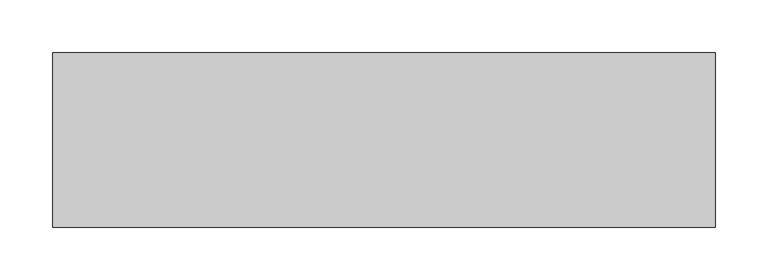
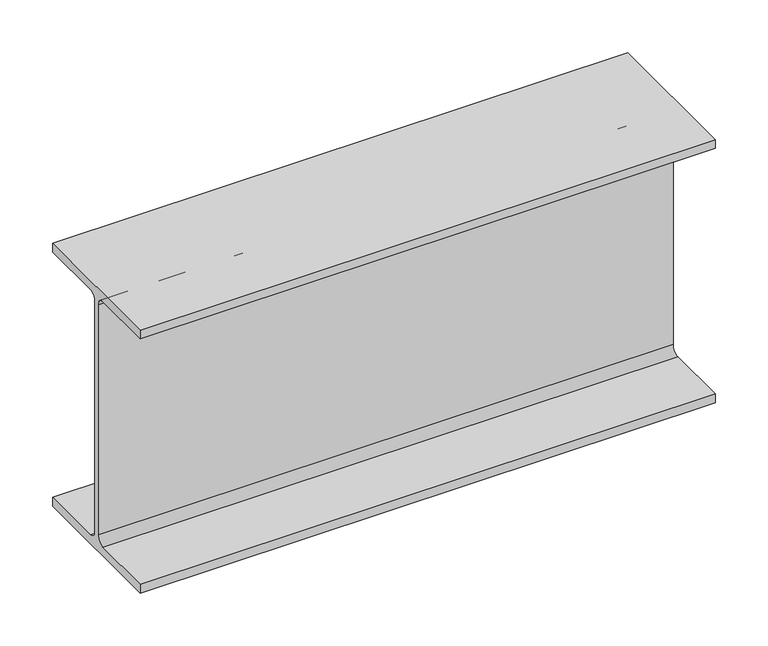
"""IFC4 building model written with IfcOpenShell, lengths in millimetres: beam geometry, Old_Steel Beam_H-KSD3502 : H_SB_ASB_H-300×150x6.5x9."""

from ifc_helpers import new_model, si_unit, point, frame, frame_2d, origin, place, context, project, spatial, polyline, circle_curve, trimmed, segment, composite_curve, outline, extrude, source, transform, mapped, element, save


def beam_ed20dfba(model_context):
    return source(origin(), model_context, "Body", "SweptSolid", [
        extrude(outline(composite_curve([segment(polyline([(82.5, -141.5), (82.5, -151.7), (-82.5, -151.7), (-82.5, -141.5), (-11.9, -141.5)]), True, "CONTINUOUS"), segment(trimmed(circle_curve(frame_2d((-11.9, -132.6)), 8.9), [point((-11.9, -141.5))], [point((-3.0, -132.6))], True, "CARTESIAN"), True, "CONTINUOUS"), segment(polyline([(-3.0, -132.6), (-3.0, 132.6)]), True, "CONTINUOUS"), segment(trimmed(circle_curve(frame_2d((-11.9, 132.6)), 8.9), [point((-3.0, 132.6))], [point((-11.9, 141.5))], True, "CARTESIAN"), True, "CONTINUOUS"), segment(polyline([(-11.9, 141.5), (-82.5, 141.5), (-82.5, 151.7), (82.5, 151.7), (82.5, 141.5), (11.9, 141.5)]), True, "CONTINUOUS"), segment(trimmed(circle_curve(frame_2d((11.9, 132.6)), 8.9), [point((11.9, 141.5))], [point((3.0, 132.6))], True, "CARTESIAN"), True, "CONTINUOUS"), segment(polyline([(3.0, 132.6), (3.0, -132.6)]), True, "CONTINUOUS"), segment(trimmed(circle_curve(frame_2d((11.9, -132.6)), 8.9), [point((3.0, -132.6))], [point((11.9, -141.5))], True, "CARTESIAN"), True, "CONTINUOUS"), segment(polyline([(11.9, -141.5), (82.5, -141.5)]), True, "CONTINUOUS")], self_intersect=False)), frame((-370.0, 0.0, 0.0), z_axis=(1.0, 0.0, 0.0), x_axis=(0.0, 1.0, 0.0)), (0.0, 0.0, 1.0), 627.2999994),
    ])


if __name__ == "__main__":
    model = new_model("IFC4")
    model_context = context("Model", 3, world=origin())
    ifc_project = project(units=[si_unit("LENGTHUNIT", "METRE", prefix="MILLI")], contexts=[model_context])
    site = spatial("IfcSite", under=ifc_project)
    building = spatial("IfcBuilding", under=site)
    placement = place(None, origin())
    beam_shape = beam_ed20dfba(model_context)
    element("IfcBeam", 1, ObjectType="Old_Steel Beam_H-KSD3502 : H_SB_ASB_H-300×150x6.5x9", at=placement, inside=building, context=model_context, shape_type="MappedRepresentation", body=[
        mapped(beam_shape, transform((0.0, 0.0, 0.0), x_axis=(1.0, 0.0, 0.0), y_axis=(0.0, 1.0, 0.0), z_axis=(0.0, 0.0, 1.0))),
    ])
    save(model, "model.ifc")

# Revit data of these elements
# Type "Old_Steel Beam_H-KSD3502 : H_SB_ASB_H-300×150x6.5x9"
#   Width = 15.0 cm
#   Web Thickness = 0.65 cm
#   Web Fillet = 1.3 cm
#   Warping Constant = 107174.0 cm⁶
#   Torsional Moment of Inertia = 9.9539 cm⁴
#   Torsional Modulus = 1.0 cm³
#   Section Area = 46.78 cm²
#   Plastic Modulus weak axis = 105.0 cm³
#   Plastic Modulus strong axis = 542.0 cm³
#   Perimeter = 1.17 m²/m
#   Nominal Weight = 36.70 kgf/m
#   Moment of Inertia weak axis = 508.00 cm⁴
#   Moment of Inertia strong axis = 7210.00 cm⁴
#   Height = 30.0 cm
#   Flange Thickness = 0.9 cm
#   Elastic Modulus weak axis = 67.7 cm³
#   Elastic Modulus strong axis = 481.0 cm³
#   Centroid Vertical = 15.0 cm
#   Centroid Horizontal = 7.5 cm
#   Length [instance default] = 1.5240 m
#   Structural Material [instance default] = Steel, 45-345
#   Assembly Code = ""
# Element 1 (IfcBeam, "Old_Steel Beam_H-KSD3502 : H_SB_ASB_H-300×150x6.5x9")
#   Structural Material = none
# Materials
#   "Steel, 45-345": class "Metal", colour RGB 189 187 185, transparency 0, Description = "Steel 345 MPa", Cost = 0
